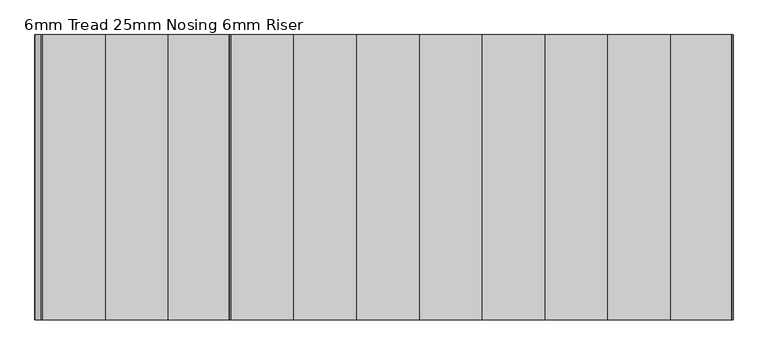
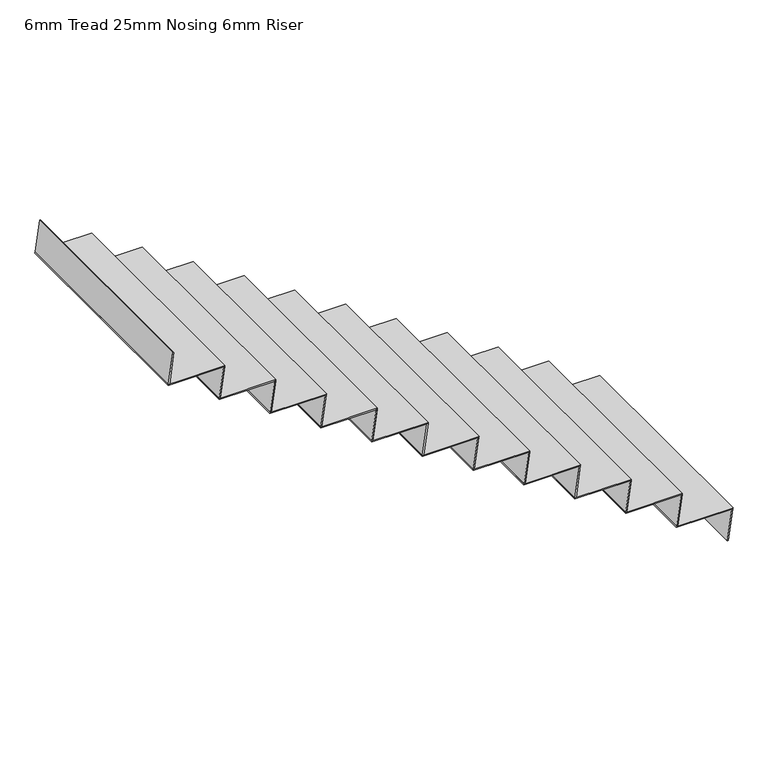
"""IFC4 building model written with IfcOpenShell, lengths in millimetres: stair flight geometry, 6mm Tread 25mm Nosing 6mm Riser."""

from ifc_helpers import new_model, si_unit, origin, place, context, project, spatial, faceted_brep, source, transform, mapped, element, save


def stair_flight_6mm_tread_25mm_nosing_6mm_riser_6fd28c6e(model_context):
    return source(origin(), model_context, "Body", "Brep", [
        faceted_brep([(-13631.0590357, 11470.4345331, 4266.6666667), (-13631.9027857, 11470.4345331, 4260.6666667), (-13631.9027857, 10220.4345331, 4260.6666667), (-13631.0590357, 10220.4345331, 4266.6666667), (-13325.0, 10220.4345331, 4266.6666667), (-13325.0, 11470.4345331, 4266.6666667), (-13325.84375, 11470.4345331, 4260.6666667), (-13325.84375, 10220.4345331, 4260.6666667)], [[[0, 1, 2, 3]], [[3, 4, 5, 0]], [[2, 1, 6, 7]], [[4, 3, 2, 7]], [[0, 5, 6, 1]], [[5, 4, 7, 6]]]),
        faceted_brep([(-13325.84375, 11470.4345331, 4260.6666667), (-13350.0, 11470.4345331, 4088.8888889), (-13356.0590357, 11470.4345331, 4088.8888889), (-13331.9027857, 11470.4345331, 4260.6666667), (-13325.84375, 10220.4345331, 4260.6666667), (-13331.9027857, 10220.4345331, 4260.6666667), (-13356.0590357, 10220.4345331, 4088.8888889), (-13350.0, 10220.4345331, 4088.8888889)], [[[0, 1, 2, 3]], [[4, 5, 6, 7]], [[1, 0, 4, 7]], [[2, 1, 7, 6]], [[3, 2, 6, 5]], [[0, 3, 5, 4]]]),
        faceted_brep([(-13600.84375, 11470.4345331, 4438.4444444), (-13625.0, 11470.4345331, 4266.6666667), (-13631.0590357, 11470.4345331, 4266.6666667), (-13606.9027857, 11470.4345331, 4438.4444444), (-13600.84375, 10220.4345331, 4438.4444444), (-13606.9027857, 10220.4345331, 4438.4444444), (-13631.0590357, 10220.4345331, 4266.6666667), (-13625.0, 10220.4345331, 4266.6666667)], [[[0, 1, 2, 3]], [[4, 5, 6, 7]], [[1, 0, 4, 7]], [[2, 1, 7, 6]], [[3, 2, 6, 5]], [[0, 3, 5, 4]]]),
        faceted_brep([(-13906.0590357, 10220.4345331, 4444.4444444), (-13600.0, 10220.4345331, 4444.4444444), (-13600.0, 11470.4345331, 4444.4444444), (-13906.0590357, 11470.4345331, 4444.4444444), (-13906.9027857, 10220.4345331, 4438.4444444), (-13906.9027857, 11470.4345331, 4438.4444444), (-13600.84375, 11470.4345331, 4438.4444444), (-13600.84375, 10220.4345331, 4438.4444444)], [[[0, 1, 2, 3]], [[4, 5, 6, 7]], [[1, 0, 4, 7]], [[3, 2, 6, 5]], [[3, 5, 4, 0]], [[2, 1, 7, 6]]]),
        faceted_brep([(-13875.84375, 11470.4345331, 4616.2222222), (-13900.0, 11470.4345331, 4444.4444444), (-13906.0590357, 11470.4345331, 4444.4444444), (-13881.9027857, 11470.4345331, 4616.2222222), (-13875.84375, 10220.4345331, 4616.2222222), (-13881.9027857, 10220.4345331, 4616.2222222), (-13906.0590357, 10220.4345331, 4444.4444444), (-13900.0, 10220.4345331, 4444.4444444)], [[[0, 1, 2, 3]], [[4, 5, 6, 7]], [[1, 0, 4, 7]], [[2, 1, 7, 6]], [[3, 2, 6, 5]], [[0, 3, 5, 4]]]),
        faceted_brep([(-14181.0590357, 10220.4345331, 4622.2222222), (-13875.0, 10220.4345331, 4622.2222222), (-13875.0, 11470.4345331, 4622.2222222), (-14181.0590357, 11470.4345331, 4622.2222222), (-14181.9027857, 10220.4345331, 4616.2222222), (-14181.9027857, 11470.4345331, 4616.2222222), (-13875.84375, 11470.4345331, 4616.2222222), (-13875.84375, 10220.4345331, 4616.2222222)], [[[0, 1, 2, 3]], [[4, 5, 6, 7]], [[1, 0, 4, 7]], [[3, 2, 6, 5]], [[3, 5, 4, 0]], [[2, 1, 7, 6]]]),
        faceted_brep([(-14150.84375, 11470.4345331, 4794.0), (-14175.0, 11470.4345331, 4622.2222222), (-14181.0590357, 11470.4345331, 4622.2222222), (-14156.9027857, 11470.4345331, 4794.0), (-14150.84375, 10220.4345331, 4794.0), (-14156.9027857, 10220.4345331, 4794.0), (-14181.0590357, 10220.4345331, 4622.2222222), (-14175.0, 10220.4345331, 4622.2222222)], [[[0, 1, 2, 3]], [[4, 5, 6, 7]], [[1, 0, 4, 7]], [[2, 1, 7, 6]], [[3, 2, 6, 5]], [[0, 3, 5, 4]]]),
        faceted_brep([(-14456.0590357, 10220.4345331, 4800.0), (-14150.0, 10220.4345331, 4800.0), (-14150.0, 11470.4345331, 4800.0), (-14456.0590357, 11470.4345331, 4800.0), (-14456.9027857, 10220.4345331, 4794.0), (-14456.9027857, 11470.4345331, 4794.0), (-14150.84375, 11470.4345331, 4794.0), (-14150.84375, 10220.4345331, 4794.0)], [[[0, 1, 2, 3]], [[4, 5, 6, 7]], [[1, 0, 4, 7]], [[3, 2, 6, 5]], [[3, 5, 4, 0]], [[2, 1, 7, 6]]]),
        faceted_brep([(-14425.84375, 11470.4345331, 4971.7777778), (-14450.0, 11470.4345331, 4800.0), (-14456.0590357, 11470.4345331, 4800.0), (-14431.9027857, 11470.4345331, 4971.7777778), (-14425.84375, 10220.4345331, 4971.7777778), (-14431.9027857, 10220.4345331, 4971.7777778), (-14456.0590357, 10220.4345331, 4800.0), (-14450.0, 10220.4345331, 4800.0)], [[[0, 1, 2, 3]], [[4, 5, 6, 7]], [[1, 0, 4, 7]], [[2, 1, 7, 6]], [[3, 2, 6, 5]], [[0, 3, 5, 4]]]),
        faceted_brep([(-14731.0590357, 10220.4345331, 4977.7777778), (-14425.0, 10220.4345331, 4977.7777778), (-14425.0, 11470.4345331, 4977.7777778), (-14731.0590357, 11470.4345331, 4977.7777778), (-14731.9027857, 10220.4345331, 4971.7777778), (-14731.9027857, 11470.4345331, 4971.7777778), (-14425.84375, 11470.4345331, 4971.7777778), (-14425.84375, 10220.4345331, 4971.7777778)], [[[0, 1, 2, 3]], [[4, 5, 6, 7]], [[1, 0, 4, 7]], [[3, 2, 6, 5]], [[3, 5, 4, 0]], [[2, 1, 7, 6]]]),
        faceted_brep([(-14700.84375, 11470.4345331, 5149.5555556), (-14725.0, 11470.4345331, 4977.7777778), (-14731.0590357, 11470.4345331, 4977.7777778), (-14706.9027857, 11470.4345331, 5149.5555556), (-14700.84375, 10220.4345331, 5149.5555556), (-14706.9027857, 10220.4345331, 5149.5555556), (-14731.0590357, 10220.4345331, 4977.7777778), (-14725.0, 10220.4345331, 4977.7777778)], [[[0, 1, 2, 3]], [[4, 5, 6, 7]], [[1, 0, 4, 7]], [[2, 1, 7, 6]], [[3, 2, 6, 5]], [[0, 3, 5, 4]]]),
        faceted_brep([(-15006.0590357, 10220.4345331, 5155.5555556), (-14700.0, 10220.4345331, 5155.5555556), (-14700.0, 11470.4345331, 5155.5555556), (-15006.0590357, 11470.4345331, 5155.5555556), (-15006.9027857, 10220.4345331, 5149.5555556), (-15006.9027857, 11470.4345331, 5149.5555556), (-14700.84375, 11470.4345331, 5149.5555556), (-14700.84375, 10220.4345331, 5149.5555556)], [[[0, 1, 2, 3]], [[4, 5, 6, 7]], [[1, 0, 4, 7]], [[3, 2, 6, 5]], [[3, 5, 4, 0]], [[2, 1, 7, 6]]]),
        faceted_brep([(-14975.84375, 11470.4345331, 5327.3333333), (-15000.0, 11470.4345331, 5155.5555556), (-15006.0590357, 11470.4345331, 5155.5555556), (-14981.9027857, 11470.4345331, 5327.3333333), (-14975.84375, 10220.4345331, 5327.3333333), (-14981.9027857, 10220.4345331, 5327.3333333), (-15006.0590357, 10220.4345331, 5155.5555556), (-15000.0, 10220.4345331, 5155.5555556)], [[[0, 1, 2, 3]], [[4, 5, 6, 7]], [[1, 0, 4, 7]], [[2, 1, 7, 6]], [[3, 2, 6, 5]], [[0, 3, 5, 4]]]),
        faceted_brep([(-15281.0590357, 10220.4345331, 5333.3333333), (-14975.0, 10220.4345331, 5333.3333333), (-14975.0, 11470.4345331, 5333.3333333), (-15281.0590357, 11470.4345331, 5333.3333333), (-15281.9027857, 10220.4345331, 5327.3333333), (-15281.9027857, 11470.4345331, 5327.3333333), (-14975.84375, 11470.4345331, 5327.3333333), (-14975.84375, 10220.4345331, 5327.3333333)], [[[0, 1, 2, 3]], [[4, 5, 6, 7]], [[1, 0, 4, 7]], [[3, 2, 6, 5]], [[3, 5, 4, 0]], [[2, 1, 7, 6]]]),
        faceted_brep([(-15250.84375, 11470.4345331, 5505.1111111), (-15275.0, 11470.4345331, 5333.3333333), (-15281.0590357, 11470.4345331, 5333.3333333), (-15256.9027857, 11470.4345331, 5505.1111111), (-15250.84375, 10220.4345331, 5505.1111111), (-15256.9027857, 10220.4345331, 5505.1111111), (-15281.0590357, 10220.4345331, 5333.3333333), (-15275.0, 10220.4345331, 5333.3333333)], [[[0, 1, 2, 3]], [[4, 5, 6, 7]], [[1, 0, 4, 7]], [[2, 1, 7, 6]], [[3, 2, 6, 5]], [[0, 3, 5, 4]]]),
        faceted_brep([(-15556.0590357, 10220.4345331, 5511.1111111), (-15250.0, 10220.4345331, 5511.1111111), (-15250.0, 11470.4345331, 5511.1111111), (-15556.0590357, 11470.4345331, 5511.1111111), (-15556.9027857, 10220.4345331, 5505.1111111), (-15556.9027857, 11470.4345331, 5505.1111111), (-15250.84375, 11470.4345331, 5505.1111111), (-15250.84375, 10220.4345331, 5505.1111111)], [[[0, 1, 2, 3]], [[4, 5, 6, 7]], [[1, 0, 4, 7]], [[3, 2, 6, 5]], [[3, 5, 4, 0]], [[2, 1, 7, 6]]]),
        faceted_brep([(-15525.84375, 11470.4345331, 5682.8888889), (-15550.0, 11470.4345331, 5511.1111111), (-15556.0590357, 11470.4345331, 5511.1111111), (-15531.9027857, 11470.4345331, 5682.8888889), (-15525.84375, 10220.4345331, 5682.8888889), (-15531.9027857, 10220.4345331, 5682.8888889), (-15556.0590357, 10220.4345331, 5511.1111111), (-15550.0, 10220.4345331, 5511.1111111)], [[[0, 1, 2, 3]], [[4, 5, 6, 7]], [[1, 0, 4, 7]], [[2, 1, 7, 6]], [[3, 2, 6, 5]], [[0, 3, 5, 4]]]),
        faceted_brep([(-15831.0590357, 10220.4345331, 5688.8888889), (-15525.0, 10220.4345331, 5688.8888889), (-15525.0, 11470.4345331, 5688.8888889), (-15831.0590357, 11470.4345331, 5688.8888889), (-15831.9027857, 10220.4345331, 5682.8888889), (-15831.9027857, 11470.4345331, 5682.8888889), (-15525.84375, 11470.4345331, 5682.8888889), (-15525.84375, 10220.4345331, 5682.8888889)], [[[0, 1, 2, 3]], [[4, 5, 6, 7]], [[1, 0, 4, 7]], [[3, 2, 6, 5]], [[3, 5, 4, 0]], [[2, 1, 7, 6]]]),
        faceted_brep([(-15800.84375, 11470.4345331, 5860.6666667), (-15825.0, 11470.4345331, 5688.8888889), (-15831.0590357, 11470.4345331, 5688.8888889), (-15806.9027857, 11470.4345331, 5860.6666667), (-15800.84375, 10220.4345331, 5860.6666667), (-15806.9027857, 10220.4345331, 5860.6666667), (-15831.0590357, 10220.4345331, 5688.8888889), (-15825.0, 10220.4345331, 5688.8888889)], [[[0, 1, 2, 3]], [[4, 5, 6, 7]], [[1, 0, 4, 7]], [[2, 1, 7, 6]], [[3, 2, 6, 5]], [[0, 3, 5, 4]]]),
        faceted_brep([(-16106.0590357, 10220.4345331, 5866.6666667), (-15800.0, 10220.4345331, 5866.6666667), (-15800.0, 11470.4345331, 5866.6666667), (-16106.0590357, 11470.4345331, 5866.6666667), (-16106.9027857, 10220.4345331, 5860.6666667), (-16106.9027857, 11470.4345331, 5860.6666667), (-15800.84375, 11470.4345331, 5860.6666667), (-15800.84375, 10220.4345331, 5860.6666667)], [[[0, 1, 2, 3]], [[4, 5, 6, 7]], [[1, 0, 4, 7]], [[3, 2, 6, 5]], [[3, 5, 4, 0]], [[2, 1, 7, 6]]]),
        faceted_brep([(-16350.84375, 11470.4345331, 6216.2222222), (-16375.0, 11470.4345331, 6044.4444444), (-16381.0590357, 11470.4345331, 6044.4444444), (-16356.9027857, 11470.4345331, 6216.2222222), (-16350.84375, 10220.4345331, 6216.2222222), (-16356.9027857, 10220.4345331, 6216.2222222), (-16381.0590357, 10220.4345331, 6044.4444444), (-16375.0, 10220.4345331, 6044.4444444)], [[[0, 1, 2, 3]], [[4, 5, 6, 7]], [[1, 0, 4, 7]], [[2, 1, 7, 6]], [[3, 2, 6, 5]], [[0, 3, 5, 4]]]),
        faceted_brep([(-16075.84375, 11470.4345331, 6038.4444444), (-16100.0, 11470.4345331, 5866.6666667), (-16106.0590357, 11470.4345331, 5866.6666667), (-16081.9027857, 11470.4345331, 6038.4444444), (-16075.84375, 10220.4345331, 6038.4444444), (-16081.9027857, 10220.4345331, 6038.4444444), (-16106.0590357, 10220.4345331, 5866.6666667), (-16100.0, 10220.4345331, 5866.6666667)], [[[0, 1, 2, 3]], [[4, 5, 6, 7]], [[1, 0, 4, 7]], [[2, 1, 7, 6]], [[3, 2, 6, 5]], [[0, 3, 5, 4]]]),
        faceted_brep([(-16381.0590357, 10220.4345331, 6044.4444444), (-16350.0, 10220.4345331, 6044.4444444), (-16075.0, 10220.4345331, 6044.4444444), (-16075.0, 11470.4345331, 6044.4444444), (-16381.0590357, 11470.4345331, 6044.4444444), (-16381.9027857, 10220.4345331, 6038.4444444), (-16381.9027857, 11470.4345331, 6038.4444444), (-16075.84375, 11470.4345331, 6038.4444444), (-16075.84375, 10220.4345331, 6038.4444444), (-16350.0, 10220.4345331, 6038.4444444)], [[[0, 1, 2, 3, 4]], [[5, 6, 7, 8, 9]], [[1, 0, 5, 9]], [[2, 1, 9, 8]], [[4, 3, 7, 6]], [[4, 6, 5, 0]], [[3, 2, 8, 7]]]),
    ])


if __name__ == "__main__":
    model = new_model("IFC4")
    model_context = context("Model", 3, world=origin())
    ifc_project = project(units=[si_unit("LENGTHUNIT", "METRE", prefix="MILLI")], contexts=[model_context])
    site = spatial("IfcSite", under=ifc_project)
    building = spatial("IfcBuilding", under=site)
    placement = place(None, origin())
    stair_flight_6mm_tread_25mm_nosing_6mm_riser_shape = stair_flight_6mm_tread_25mm_nosing_6mm_riser_6fd28c6e(model_context)
    element("IfcStairFlight", 1, ObjectType="6mm Tread 25mm Nosing 6mm Riser", at=placement, inside=building, context=model_context, shape_type="MappedRepresentation", body=[
        mapped(stair_flight_6mm_tread_25mm_nosing_6mm_riser_shape, transform((0.0, 0.0, 0.0), x_axis=(1.0, 0.0, 0.0), y_axis=(0.0, 1.0, 0.0), z_axis=(0.0, 0.0, 1.0))),
    ])
    save(model, "model.ifc")

# Revit data of these elements
# Element 1 (IfcStairFlight, "6mm Tread 25mm Nosing 6mm Riser")
#   Materials on its faces: "Steel, Paint Finish, Dark Gray"
# Materials
#   "Steel, Paint Finish, Dark Gray": class "Metal", colour RGB 89 89 89, transparency 0, Description = "Steel, paint finish, dark gray, glossy", Cost = 0
